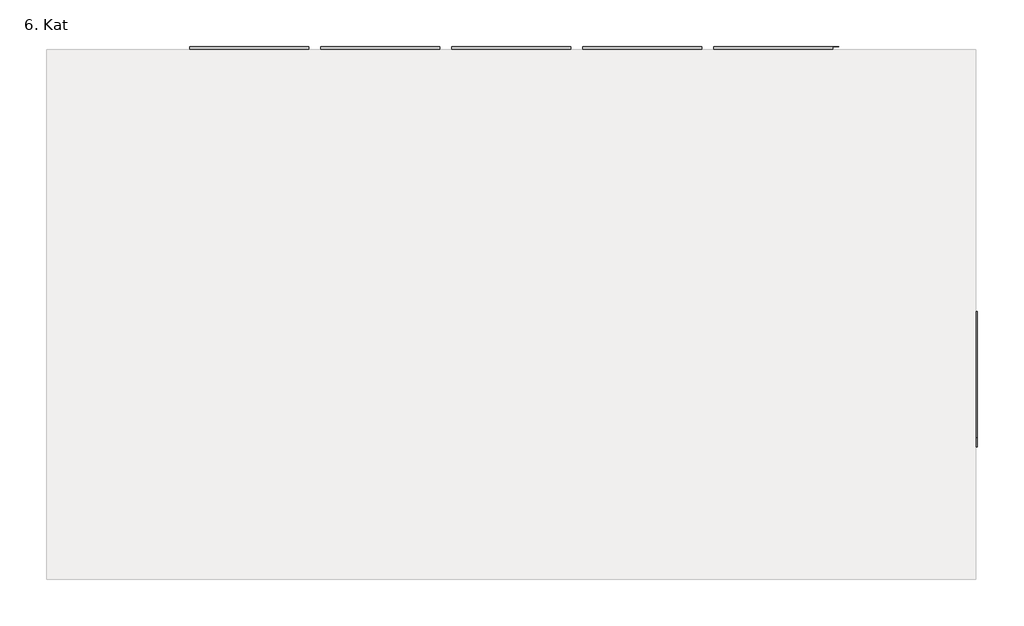
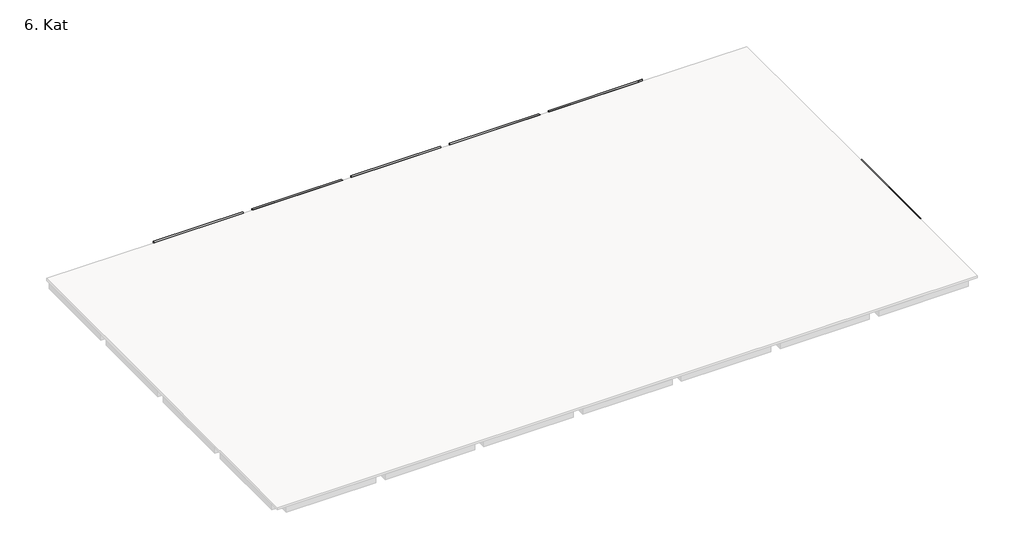
# One storey, part 2 of 2: 40 beams.
"""IFC4 building model written with IfcOpenShell, lengths in millimetres."""

from ifc_helpers import new_model, si_unit, frame, origin, place, context, project, spatial, polyline, outline, extrude, faceted_brep, element, save

model = new_model("IFC4")

# Units and contexts
model_context = context("Model", 3, world=origin())
ifc_project = project(units=[si_unit("LENGTHUNIT", "METRE", prefix="MILLI")], contexts=[model_context])

# Site, building, storey
site = spatial("IfcSite", under=ifc_project)
building = spatial("IfcBuilding", under=site)
storey = spatial("IfcBuildingStorey", under=building, Name="6. Kat", Elevation=31100.0)

# Beams
placement = place(None, origin())
element("IfcBeam", 1, ObjectType="M_Concrete-Rectangular Beam : 60x70cm kiriş", at=placement, inside=storey, context=model_context, shape_type="Brep", body=[
    faceted_brep([(16599.9993907, 34000.0004302, 31100.0), (16599.9993907, 34200.0000099, 31100.0), (8899.9995273, 34200.0000099, 31100.0), (8899.9995273, 34000.0004302, 31100.0), (8899.9993907, 33600.0000099, 30900.0), (8899.9993907, 33600.0000099, 30400.0), (16599.9993907, 33600.0000099, 30400.0), (16599.9993907, 33600.0000099, 30900.0), (8899.9995273, 34200.0000099, 30400.0), (16599.9993907, 34200.0000099, 30400.0), (8899.9993907, 34000.0004302, 30900.0), (16599.9993907, 34000.0004302, 30900.0)], [[[0, 1, 2, 3]], [[4, 5, 6, 7]], [[5, 8, 9, 6]], [[1, 9, 8, 2]], [[5, 4, 10, 3, 2, 8]], [[4, 7, 11, 10]], [[6, 9, 1, 0, 11, 7]], [[10, 11, 0, 3]]]),
])
element("IfcBeam", 2, ObjectType="M_Concrete-Rectangular Beam : 60x70cm kiriş", at=placement, inside=storey, context=model_context, shape_type="Brep", body=[
    faceted_brep([(25099.9993907, 34000.0004302, 31100.0), (25099.9993907, 34200.0000277, 31100.0), (17399.9993907, 34200.0000277, 31100.0), (17399.9993907, 34000.0004302, 31100.0), (25099.9993907, 33600.0000277, 30900.0), (17399.9996817, 33600.0000277, 30900.0), (17399.9996817, 33600.0000277, 30400.0), (25099.9993907, 33600.0000277, 30400.0), (17399.9993907, 34200.0000277, 30400.0), (25099.9993907, 34200.0000277, 30400.0), (17399.9993907, 34000.0004302, 30900.0), (25099.9993907, 34000.0004302, 30900.0)], [[[0, 1, 2, 3]], [[4, 5, 6, 7]], [[7, 6, 8, 9]], [[1, 9, 8, 2]], [[10, 5, 4, 11]], [[11, 0, 3, 10]], [[6, 5, 10, 3, 2, 8]], [[7, 9, 1, 0, 11, 4]]]),
])
element("IfcBeam", 3, ObjectType="M_Concrete-Rectangular Beam : 60x70cm kiriş", at=placement, inside=storey, context=model_context, shape_type="Brep", body=[
    faceted_brep([(33599.9993907, 34000.0004302, 31100.0), (33599.9993907, 34200.000044, 31100.0), (25899.9993907, 34200.000044, 31100.0), (25899.9993907, 34000.0004302, 31100.0), (33599.9993907, 34200.000044, 30400.0), (25899.9993907, 34200.000044, 30400.0), (25899.9996503, 33600.000044, 30400.0), (33599.9993907, 33600.000044, 30400.0), (25899.9996503, 33600.000044, 30900.0), (33599.9993907, 33600.000044, 30900.0), (25899.9993907, 34000.0004302, 30900.0), (33599.9993907, 34000.0004302, 30900.0)], [[[0, 1, 2, 3]], [[1, 4, 5, 2]], [[6, 5, 4, 7]], [[8, 6, 7, 9]], [[10, 8, 9, 11]], [[11, 0, 3, 10]], [[6, 8, 10, 3, 2, 5]], [[1, 0, 11, 9, 7, 4]]]),
])
element("IfcBeam", 4, ObjectType="M_Concrete-Rectangular Beam : 60x70cm kiriş", at=placement, inside=storey, context=model_context, shape_type="SweptSolid", body=[
    extrude(outline(polyline([(34200.0000618, 31100.0), (34200.0000618, 30400.0), (33600.0000618, 30400.0), (33600.0000618, 30900.0), (34000.0004302, 30900.0), (34000.0004302, 31100.0), (34200.0000618, 31100.0)])), frame((34399.9993907, 0.0, 0.0), z_axis=(1.0, 0.0, 0.0), x_axis=(0.0, 1.0, 0.0)), (0.0, 0.0, 1.0), 7699.9999993),
])
element("IfcBeam", 5, ObjectType="M_Concrete-Rectangular Beam : 60x70cm kiriş", at=placement, inside=storey, context=model_context, shape_type="Brep", body=[
    faceted_brep([(50999.9994944, 34200.0000788, 31100.0), (42899.999681, 34200.0000788, 31100.0), (42899.999681, 34000.0004302, 31100.0), (50599.9994944, 34000.0004302, 31100.0), (50599.9994944, 34193.7257565, 31100.0), (50999.9994944, 34193.7257565, 31100.0), (42899.999681, 34200.0000788, 30400.0), (50999.9994944, 34200.0000788, 30400.0), (42899.999681, 33600.0000788, 30400.0), (50999.9994944, 34193.7257565, 30400.0), (50599.9994944, 34193.7257565, 30400.0), (50599.9994944, 33600.0000788, 30400.0), (42899.999681, 33600.0000788, 30900.0), (50599.9994944, 33600.0000788, 30900.0), (42899.999681, 34000.0004302, 30900.0), (50599.9994944, 34000.0004302, 30900.0)], [[[0, 1, 2, 3, 4, 5]], [[6, 1, 0, 7]], [[8, 6, 7, 9, 10, 11]], [[12, 8, 11, 13]], [[14, 12, 13, 15]], [[2, 14, 15, 3]], [[1, 6, 8, 12, 14, 2]], [[7, 0, 5, 9]], [[10, 4, 3, 15, 13, 11]], [[4, 10, 9, 5]]]),
])
element("IfcBeam", 6, ObjectType="M_Concrete-Rectangular Beam : 60x70cm kiriş", at=placement, inside=storey, context=model_context, shape_type="SweptSolid", body=[
    extrude(outline(polyline([(16799.9996817, 33600.0009197), (17399.9996817, 33600.0009197), (17399.9996817, 25900.0003816), (16799.9996817, 25900.0003816), (16799.9996817, 33600.0009197)])), frame((0.0, 0.0, 30400.0), z_axis=(0.0, 0.0, 1.0), x_axis=(1.0, 0.0, 0.0)), (0.0, 0.0, 1.0), 500.0),
])
element("IfcBeam", 7, ObjectType="M_Concrete-Rectangular Beam : 60x70cm kiriş", at=placement, inside=storey, context=model_context, shape_type="SweptSolid", body=[
    extrude(outline(polyline([(25899.9996503, 25900.0004105), (25299.9996503, 25900.0004105), (25299.9996503, 33600.0009197), (25899.9996503, 33600.0009197), (25899.9996503, 25900.0004105)])), frame((0.0, 0.0, 30400.0), z_axis=(0.0, 0.0, 1.0), x_axis=(1.0, 0.0, 0.0)), (0.0, 0.0, 1.0), 500.0),
])
element("IfcBeam", 8, ObjectType="M_Concrete-Rectangular Beam : 60x70cm kiriş", at=placement, inside=storey, context=model_context, shape_type="Brep", body=[
    faceted_brep([(17399.9996817, 25900.0000279, 30400.0), (17399.9996817, 25900.0000279, 30900.0), (25099.9993907, 25900.0000279, 30900.0), (25099.9993907, 25900.0000279, 30400.0), (17399.9995362, 25300.0000279, 30400.0), (25099.9993907, 25300.0000279, 30400.0), (25099.9993907, 25300.0000279, 30900.0), (17399.9995362, 25300.0000279, 30900.0)], [[[0, 1, 2, 3]], [[4, 0, 3, 5]], [[5, 6, 7, 4]], [[4, 7, 1, 0]], [[2, 1, 7, 6]], [[5, 3, 2, 6]]]),
])
element("IfcBeam", 9, ObjectType="M_Concrete-Rectangular Beam : 60x70cm kiriş", at=placement, inside=storey, context=model_context, shape_type="SweptSolid", body=[
    extrude(outline(polyline([(25299.999682, 25099.9999518), (25899.999682, 25099.9999518), (25899.999682, 17400.0009197), (25299.999682, 17400.0009197), (25299.999682, 25099.9999518)])), frame((0.0, 0.0, 30400.0), z_axis=(0.0, 0.0, 1.0), x_axis=(1.0, 0.0, 0.0)), (0.0, 0.0, 1.0), 500.0),
])
element("IfcBeam", 10, ObjectType="M_Concrete-Rectangular Beam : 60x70cm kiriş", at=placement, inside=storey, context=model_context, shape_type="Brep", body=[
    faceted_brep([(25899.9996503, 25900.0003995, 30400.0), (25899.9996503, 25900.0003995, 30900.0), (33599.9993907, 25900.0003995, 30900.0), (33599.9993907, 25900.0003995, 30400.0), (25899.9993907, 25300.0003995, 30400.0), (33599.9993907, 25300.0003995, 30400.0), (25899.9993907, 25300.0003995, 30900.0), (33599.9993907, 25300.0003995, 30900.0)], [[[0, 1, 2, 3]], [[4, 0, 3, 5]], [[6, 4, 5, 7]], [[1, 0, 4, 6]], [[1, 6, 7, 2]], [[3, 2, 7, 5]]]),
])
element("IfcBeam", 11, ObjectType="M_Concrete-Rectangular Beam : 60x70cm kiriş", at=placement, inside=storey, context=model_context, shape_type="Brep", body=[
    faceted_brep([(33599.9994248, 33600.000044, 30900.0), (33599.9994248, 33600.000044, 30400.0), (33599.9994248, 25900.0003995, 30400.0), (33599.9994248, 25900.0003995, 30900.0), (34199.9994248, 33600.0009197, 30400.0), (34199.9994248, 25900.0004105, 30400.0), (34199.9994248, 25900.0004105, 30900.0), (34199.9994248, 33600.0009197, 30900.0)], [[[0, 1, 2, 3]], [[1, 4, 5, 2]], [[6, 5, 4, 7]], [[1, 0, 7, 4]], [[3, 2, 5, 6]], [[7, 0, 3, 6]]]),
])
element("IfcBeam", 12, ObjectType="M_Concrete-Rectangular Beam : 60x70cm kiriş", at=placement, inside=storey, context=model_context, shape_type="SweptSolid", body=[
    extrude(outline(polyline([(34399.9993907, 25300.0004179), (34399.9993907, 25900.0004179), (42099.9995162, 25900.0004179), (42099.9995162, 25300.0004179), (34399.9993907, 25300.0004179)])), frame((0.0, 0.0, 30400.0), z_axis=(0.0, 0.0, 1.0), x_axis=(1.0, 0.0, 0.0)), (0.0, 0.0, 1.0), 500.0),
])
element("IfcBeam", 13, ObjectType="M_Concrete-Rectangular Beam : 60x70cm kiriş", at=placement, inside=storey, context=model_context, shape_type="Brep", body=[
    faceted_brep([(42099.9994393, 25900.0004179, 30400.0), (42099.9994393, 25900.0004179, 30900.0), (42099.9994393, 33600.0000618, 30900.0), (42099.9994393, 33600.0000618, 30400.0), (42699.9994393, 25900.0004459, 30400.0), (42699.9994393, 33600.0009197, 30400.0), (42699.9994393, 33600.0009197, 30900.0), (42699.9994393, 25900.0004459, 30900.0)], [[[0, 1, 2, 3]], [[4, 0, 3, 5]], [[5, 6, 7, 4]], [[4, 7, 1, 0]], [[3, 2, 6, 5]], [[2, 1, 7, 6]]]),
])
element("IfcBeam", 14, ObjectType="M_Concrete-Rectangular Beam : 60x70cm kiriş", at=placement, inside=storey, context=model_context, shape_type="SweptSolid", body=[
    extrude(outline(polyline([(50599.9993899, 25900.0004722), (50599.9993899, 25300.0004722), (47199.999381, 25300.0004722), (47199.999381, 25900.0004722), (50599.9993899, 25900.0004722)])), frame((0.0, 0.0, 30400.0), z_axis=(0.0, 0.0, 1.0), x_axis=(1.0, 0.0, 0.0)), (0.0, 0.0, 1.0), 500.0),
])
element("IfcBeam", 15, ObjectType="M_Concrete-Rectangular Beam : 60x70cm kiriş", at=placement, inside=storey, context=model_context, shape_type="Brep", body=[
    faceted_brep([(51199.9994348, 25899.9999188, 30900.0), (51199.9994348, 25899.9999188, 30400.0), (51199.9994348, 33600.0004303, 30400.0), (51199.9994348, 33600.0004303, 30900.0), (50599.9994348, 33600.0000788, 30400.0), (50599.9994348, 25900.0004722, 30400.0), (50599.9994348, 33600.0000788, 30900.0), (50599.9994348, 25900.0004722, 30900.0)], [[[0, 1, 2, 3]], [[4, 2, 1, 5]], [[6, 4, 5, 7]], [[4, 6, 3, 2]], [[7, 5, 1, 0]], [[3, 6, 7, 0]]]),
])
element("IfcBeam", 16, ObjectType="M_Concrete-Rectangular Beam : 60x70cm kiriş", at=placement, inside=storey, context=model_context, shape_type="SweptSolid", body=[
    extrude(outline(polyline([(59100.0000836, 25300.0000972), (51399.9996879, 25300.0000972), (51399.9996879, 25900.0000972), (59100.0000836, 25900.0000972), (59100.0000836, 25300.0000972)])), frame((0.0, 0.0, 30400.0), z_axis=(0.0, 0.0, 1.0), x_axis=(1.0, 0.0, 0.0)), (0.0, 0.0, 1.0), 500.0),
])
element("IfcBeam", 17, ObjectType="M_Concrete-Rectangular Beam : 60x70cm kiriş", at=placement, inside=storey, context=model_context, shape_type="SweptSolid", body=[
    extrude(outline(polyline([(59899.9996867, 25900.0004522), (59299.9996867, 25900.0004522), (59299.9996867, 33600.0004303), (59899.9996867, 33600.0004303), (59899.9996867, 25900.0004522)])), frame((0.0, 0.0, 30400.0), z_axis=(0.0, 0.0, 1.0), x_axis=(1.0, 0.0, 0.0)), (0.0, 0.0, 1.0), 500.0),
])
element("IfcBeam", 18, ObjectType="M_Concrete-Rectangular Beam : 60x70cm kiriş", at=placement, inside=storey, context=model_context, shape_type="SweptSolid", body=[
    extrude(outline(polyline([(33599.9994953, 25100.0004105), (34199.9994953, 25100.0004105), (34199.9994953, 17400.0009197), (33599.9994953, 17400.0009197), (33599.9994953, 25100.0004105)])), frame((0.0, 0.0, 30400.0), z_axis=(0.0, 0.0, 1.0), x_axis=(1.0, 0.0, 0.0)), (0.0, 0.0, 1.0), 500.0),
])
element("IfcBeam", 19, ObjectType="M_Concrete-Rectangular Beam : 40x70cm kiriş 2", at=placement, inside=storey, context=model_context, shape_type="SweptSolid", body=[
    extrude(outline(polyline([(42099.9995162, 16050.0004138), (42499.9995162, 16050.0004138), (42499.9995162, 14100.0003816), (42099.9995162, 14100.0003816), (42099.9995162, 16050.0004138)])), frame((0.0, 0.0, 30400.0), z_axis=(0.0, 0.0, 1.0), x_axis=(1.0, 0.0, 0.0)), (0.0, 0.0, 1.0), 500.0),
])
element("IfcBeam", 20, ObjectType="M_Concrete-Rectangular Beam : 40x70cm kiriş 2", at=placement, inside=storey, context=model_context, shape_type="SweptSolid", body=[
    extrude(outline(polyline([(41999.9997966, 13700.0003995), (41999.9997966, 13300.0003995), (34399.9997415, 13300.0003995), (34399.9997415, 13700.0003995), (41999.9997966, 13700.0003995)])), frame((0.0, 0.0, 30400.0), z_axis=(0.0, 0.0, 1.0), x_axis=(1.0, 0.0, 0.0)), (0.0, 0.0, 1.0), 500.0),
])
element("IfcBeam", 21, ObjectType="M_Concrete-Rectangular Beam : 40x70cm kiriş 2", at=placement, inside=storey, context=model_context, shape_type="SweptSolid", body=[
    extrude(outline(polyline([(34399.9993907, 17000.0007895), (34399.9993907, 17400.0007895), (42099.9995162, 17400.0007895), (42099.9995162, 17000.0007895), (34399.9993907, 17000.0007895)])), frame((0.0, 0.0, 30400.0), z_axis=(0.0, 0.0, 1.0), x_axis=(1.0, 0.0, 0.0)), (0.0, 0.0, 1.0), 500.0),
])
element("IfcBeam", 22, ObjectType="M_Concrete-Rectangular Beam : 40x70cm kiriş 2", at=placement, inside=storey, context=model_context, shape_type="SweptSolid", body=[
    extrude(outline(polyline([(42499.9995162, 17000.0003766), (42499.9995162, 17400.0003766), (46799.999381, 17400.0003766), (46799.999381, 17000.0003766), (42499.9995162, 17000.0003766)])), frame((0.0, 0.0, 30400.0), z_axis=(0.0, 0.0, 1.0), x_axis=(1.0, 0.0, 0.0)), (0.0, 0.0, 1.0), 500.0),
])
element("IfcBeam", 23, ObjectType="M_Concrete-Rectangular Beam : 60x70cm kiriş", at=placement, inside=storey, context=model_context, shape_type="SweptSolid", body=[
    extrude(outline(polyline([(33599.9997451, 14100.0003995), (33599.9997451, 16599.9999518), (34199.9997451, 16599.9999518), (34199.9997451, 14100.0003995), (33599.9997451, 14100.0003995)])), frame((0.0, 0.0, 30400.0), z_axis=(0.0, 0.0, 1.0), x_axis=(1.0, 0.0, 0.0)), (0.0, 0.0, 1.0), 500.0),
])
element("IfcBeam", 24, ObjectType="M_Concrete-Rectangular Beam : 40x70cm kiriş 2", at=placement, inside=storey, context=model_context, shape_type="Brep", body=[
    faceted_brep([(42899.9990901, 13300.0003995, 30400.0), (46799.999381, 13300.0003995, 30400.0), (47199.999381, 13300.0003995, 30400.0), (50599.9996909, 13300.0003995, 30400.0), (50599.9996909, 13300.0003995, 30900.0), (47199.999381, 13300.0003995, 30900.0), (46799.999381, 13300.0003995, 30900.0), (42899.9990901, 13300.0003995, 30900.0), (42899.9990901, 13700.0003995, 30400.0), (46799.999381, 13700.0003995, 30400.0), (47199.999381, 13700.0003995, 30400.0), (50599.9996909, 13700.0003995, 30400.0), (42899.9990901, 13700.0003995, 30900.0), (46799.999381, 13700.0003995, 30900.0), (47199.999381, 13700.0003995, 30900.0), (50599.9996909, 13700.0003995, 30900.0)], [[[0, 1, 2, 3, 4, 5, 6, 7]], [[3, 2, 1, 0, 8, 9, 10, 11]], [[11, 10, 9, 8, 12, 13, 14, 15]], [[3, 11, 15, 4]], [[7, 6, 5, 4, 15, 14, 13, 12]], [[8, 0, 7, 12]]]),
])
element("IfcBeam", 25, ObjectType="M_Concrete-Rectangular Beam : 40x70cm kiriş 2", at=placement, inside=storey, context=model_context, shape_type="SweptSolid", body=[
    extrude(outline(polyline([(46799.999381, 16050.0004138), (47199.999381, 16050.0004138), (47199.999381, 13700.0003995), (46799.999381, 13700.0003995), (46799.999381, 16050.0004138)])), frame((0.0, 0.0, 30400.0), z_axis=(0.0, 0.0, 1.0), x_axis=(1.0, 0.0, 0.0)), (0.0, 0.0, 1.0), 500.0),
    extrude(outline(polyline([(46799.999381, 13300.0003995), (47199.999381, 13300.0003995), (47199.999381, 8800.0009197), (46799.999381, 8800.0009197), (46799.999381, 13300.0003995)])), frame((0.0, 0.0, 30400.0), z_axis=(0.0, 0.0, 1.0), x_axis=(1.0, 0.0, 0.0)), (0.0, 0.0, 1.0), 500.0),
])
element("IfcBeam", 26, ObjectType="M_Concrete-Rectangular Beam : 60x70cm kiriş", at=placement, inside=storey, context=model_context, shape_type="Brep", body=[
    faceted_brep([(34399.9993907, 8200.0009197, 30900.0), (34399.9993907, 8200.0009197, 30400.0), (42099.9993899, 8200.0009197, 30400.0), (42099.9993899, 8200.0009197, 30900.0), (34399.9993907, 8800.0009197, 30400.0), (41999.9997966, 8800.0009197, 30400.0), (42099.9993899, 8800.0009197, 30400.0), (34399.9993907, 8800.0009197, 30900.0), (41999.9997966, 8800.0009197, 30900.0), (42099.9993899, 8800.0009197, 30900.0)], [[[0, 1, 2, 3]], [[1, 4, 5, 6, 2]], [[4, 7, 8, 9, 6, 5]], [[7, 0, 3, 9, 8]], [[1, 0, 7, 4]], [[3, 2, 6, 9]]]),
])
element("IfcBeam", 27, ObjectType="M_Concrete-Rectangular Beam : 60x70cm kiriş", at=placement, inside=storey, context=model_context, shape_type="Brep", body=[
    faceted_brep([(50599.9993899, 8200.0009197, 30400.0), (50599.9993899, 8200.0009197, 30900.0), (42899.9993899, 8200.0009197, 30900.0), (42899.9993899, 8200.0009197, 30400.0), (50599.9993899, 8800.0009197, 30400.0), (42899.9993899, 8800.0009197, 30400.0), (46799.999381, 8800.0009197, 30400.0), (47199.999381, 8800.0009197, 30400.0), (50599.9993899, 8800.0009197, 30900.0), (42899.9993899, 8800.0009197, 30900.0), (46799.999381, 8800.0009197, 30900.0), (47199.999381, 8800.0009197, 30900.0)], [[[0, 1, 2, 3]], [[4, 0, 3, 5, 6, 7]], [[8, 4, 7, 6, 5, 9, 10, 11]], [[1, 8, 11, 10, 9, 2]], [[1, 0, 4, 8]], [[3, 2, 9, 5]]]),
])
element("IfcBeam", 28, ObjectType="M_Concrete-Rectangular Beam : 60x70cm kiriş", at=placement, inside=storey, context=model_context, shape_type="Brep", body=[
    faceted_brep([(42599.9997966, 8900.0009197, 30900.0), (42599.9997966, 8900.0009197, 30400.0), (42599.9997966, 13300.0003816, 30400.0), (42599.9997966, 13300.0003816, 30900.0), (41999.9997966, 8800.0009197, 30400.0), (41999.9997966, 13300.0003995, 30400.0), (41999.9997966, 13700.0003995, 30400.0), (42099.9993899, 13700.0003995, 30400.0), (42099.9993899, 13300.0003816, 30400.0), (42099.9993899, 8900.0009197, 30400.0), (42099.9993899, 8800.0009197, 30400.0), (41999.9997966, 8800.0009197, 30900.0), (41999.9997966, 13300.0003995, 30900.0), (41999.9997966, 13700.0003995, 30900.0), (42099.9993899, 8800.0009197, 30900.0), (42099.9993899, 8900.0009197, 30900.0), (42099.9993899, 13300.0003816, 30900.0), (42099.9993899, 13700.0003995, 30900.0)], [[[0, 1, 2, 3]], [[4, 5, 6, 7, 8, 2, 1, 9, 10]], [[4, 11, 12, 13, 6, 5]], [[11, 4, 10, 14]], [[13, 12, 11, 14, 15, 0, 3, 16, 17]], [[6, 13, 17, 7]], [[9, 15, 14, 10]], [[15, 9, 1, 0]], [[8, 16, 3, 2]], [[16, 8, 7, 17]]]),
])
element("IfcBeam", 29, ObjectType="M_Concrete-Rectangular Beam : 60x70cm kiriş", at=placement, inside=storey, context=model_context, shape_type="SweptSolid", body=[
    extrude(outline(polyline([(33599.9994953, 13300.0003995), (34199.9994953, 13300.0003995), (34199.9994953, 8900.0009197), (33599.9994953, 8900.0009197), (33599.9994953, 13300.0003995)])), frame((0.0, 0.0, 30400.0), z_axis=(0.0, 0.0, 1.0), x_axis=(1.0, 0.0, 0.0)), (0.0, 0.0, 1.0), 500.0),
])
element("IfcBeam", 30, ObjectType="M_Concrete-Rectangular Beam : 60x70cm kiriş", at=placement, inside=storey, context=model_context, shape_type="SweptSolid", body=[
    extrude(outline(polyline([(47199.999381, 16800.0008288), (47199.999381, 17400.0008288), (50599.9993899, 17400.0008288), (50599.9993899, 16800.0008288), (47199.999381, 16800.0008288)])), frame((0.0, 0.0, 30400.0), z_axis=(0.0, 0.0, 1.0), x_axis=(1.0, 0.0, 0.0)), (0.0, 0.0, 1.0), 500.0),
])
element("IfcBeam", 31, ObjectType="M_Concrete-Rectangular Beam : 60x70cm kiriş", at=placement, inside=storey, context=model_context, shape_type="Brep", body=[
    faceted_brep([(50599.999688, 17400.0008288, 30400.0), (50599.999688, 17400.0008288, 30900.0), (50599.999688, 25099.9999414, 30900.0), (50599.999688, 25099.9999414, 30400.0), (51199.999688, 17400.0009197, 30400.0), (51199.999688, 25099.9999414, 30400.0), (51199.999688, 25099.9999414, 30900.0), (51199.999688, 17400.0009197, 30900.0)], [[[0, 1, 2, 3]], [[4, 0, 3, 5]], [[5, 6, 7, 4]], [[4, 7, 1, 0]], [[2, 1, 7, 6]], [[5, 3, 2, 6]]]),
])
element("IfcBeam", 32, ObjectType="M_Concrete-Rectangular Beam : 60x70cm kiriş", at=placement, inside=storey, context=model_context, shape_type="SweptSolid", body=[
    extrude(outline(polyline([(59299.9997153, 17400.0009197), (59299.9997153, 25099.9999188), (59899.9997153, 25099.9999188), (59899.9997153, 17400.0009197), (59299.9997153, 17400.0009197)])), frame((0.0, 0.0, 30400.0), z_axis=(0.0, 0.0, 1.0), x_axis=(1.0, 0.0, 0.0)), (0.0, 0.0, 1.0), 500.0),
])
element("IfcBeam", 33, ObjectType="M_Concrete-Rectangular Beam : 60x70cm kiriş", at=placement, inside=storey, context=model_context, shape_type="SweptSolid", body=[
    extrude(outline(polyline([(51399.9993899, 17399.9995872), (59100.0000836, 17399.9995872), (59100.0000836, 16799.9995872), (51399.9993899, 16799.9995872), (51399.9993899, 17399.9995872)])), frame((0.0, 0.0, 30400.0), z_axis=(0.0, 0.0, 1.0), x_axis=(1.0, 0.0, 0.0)), (0.0, 0.0, 1.0), 500.0),
])
element("IfcBeam", 34, ObjectType="M_Concrete-Rectangular Beam : 60x70cm kiriş", at=placement, inside=storey, context=model_context, shape_type="Brep", body=[
    faceted_brep([(50599.9996909, 16600.0009197, 30400.0), (50599.9996909, 13700.0003995, 30400.0), (50599.9996909, 13300.0003995, 30400.0), (50599.9996909, 8900.000455, 30400.0), (50599.9996909, 8900.000455, 30900.0), (50599.9996909, 13300.0003995, 30900.0), (50599.9996909, 13700.0003995, 30900.0), (50599.9996909, 16600.0009197, 30900.0), (51199.9996909, 16600.0009197, 30400.0), (51199.9996909, 8900.000455, 30400.0), (51199.9996909, 16600.0009197, 30900.0), (51199.9996909, 8900.000455, 30900.0)], [[[0, 1, 2, 3, 4, 5, 6, 7]], [[3, 2, 1, 0, 8, 9]], [[9, 8, 10, 11]], [[7, 6, 5, 4, 11, 10]], [[3, 9, 11, 4]], [[8, 0, 7, 10]]]),
])
element("IfcBeam", 35, ObjectType="M_Concrete-Rectangular Beam : 60x70cm kiriş", at=placement, inside=storey, context=model_context, shape_type="Brep", body=[
    faceted_brep([(59999.9993848, 8200.0009197, 31100.0), (59999.9993848, 8800.0009197, 31100.0), (59899.9997758, 8800.0009197, 31100.0), (59899.9997758, 8200.0009197, 31100.0), (59999.9993848, 8200.0009197, 30400.0), (59900.0000836, 8200.0009197, 30400.0), (59999.9993848, 8800.0009197, 30400.0), (59900.0000836, 8800.0009197, 30400.0)], [[[0, 1, 2, 3]], [[4, 0, 3, 5]], [[6, 4, 5, 7]], [[1, 6, 7, 2]], [[1, 0, 4, 6]], [[3, 2, 7, 5]]]),
    faceted_brep([(51399.9993899, 8800.0009197, 30900.0), (51399.9993899, 8200.0009197, 30900.0), (59100.0000836, 8200.0009197, 30900.0), (59100.0000836, 8800.0009197, 30900.0), (51399.9993899, 8800.0009197, 30400.0), (51399.9993899, 8200.0009197, 30400.0), (59100.0000836, 8200.0009197, 30400.0), (59100.0000836, 8800.0009197, 30400.0)], [[[0, 1, 2, 3]], [[4, 5, 1, 0]], [[2, 6, 7, 3]], [[1, 5, 6, 2]], [[5, 4, 7, 6]], [[4, 0, 3, 7]]]),
])
element("IfcBeam", 36, ObjectType="M_Concrete-Rectangular Beam : 60x70cm kiriş", at=placement, inside=storey, context=model_context, shape_type="Brep", body=[
    faceted_brep([(59999.9993848, 8800.0009197, 31100.0), (59999.9993848, 17000.0009197, 31100.0), (59899.9997758, 17000.0009197, 31100.0), (59899.9997758, 8800.0009197, 31100.0), (59999.9993848, 17000.0009197, 30400.0), (59999.9993848, 8800.0009197, 30400.0), (59900.0000836, 8800.0009197, 30400.0), (59900.0000836, 8900.0009197, 30400.0), (59399.9993848, 8900.0009197, 30400.0), (59399.9993848, 16600.0009197, 30400.0), (59900.0000836, 16600.0009197, 30400.0), (59900.0000836, 17000.0009197, 30400.0), (59399.9993848, 8900.0009197, 30900.0), (59399.9993848, 16600.0009197, 30900.0), (59899.9997758, 8900.0009197, 30900.0), (59899.9997758, 16600.0009197, 30900.0)], [[[0, 1, 2, 3]], [[4, 1, 0, 5]], [[4, 5, 6, 7, 8, 9, 10, 11]], [[8, 12, 13, 9]], [[5, 0, 3, 6]], [[12, 14, 15, 13]], [[11, 10, 15, 14, 7, 6, 3, 2]], [[1, 4, 11, 2]], [[7, 14, 12, 8]], [[15, 10, 9, 13]]]),
])
element("IfcBeam", 37, ObjectType="M_Concrete-Rectangular Beam : 60x70cm kiriş", at=placement, inside=storey, context=model_context, shape_type="SweptSolid", body=[
    extrude(outline(polyline([(59899.9997503, 400.0009197), (59299.9997503, 400.0009197), (59299.9997503, 8100.0009197), (59899.9997503, 8100.0009197), (59899.9997503, 400.0009197)])), frame((0.0, 0.0, 30400.0), z_axis=(0.0, 0.0, 1.0), x_axis=(1.0, 0.0, 0.0)), (0.0, 0.0, 1.0), 500.0),
])
element("IfcBeam", 38, ObjectType="M_Concrete-Rectangular Beam : 60x70cm kiriş", at=placement, inside=storey, context=model_context, shape_type="SweptSolid", body=[
    extrude(outline(polyline([(51199.999723, 400.0009197), (50599.999723, 400.0009197), (50599.999723, 8100.0009197), (51199.999723, 8100.0009197), (51199.999723, 400.0009197)])), frame((0.0, 0.0, 30400.0), z_axis=(0.0, 0.0, 1.0), x_axis=(1.0, 0.0, 0.0)), (0.0, 0.0, 1.0), 500.0),
])
element("IfcBeam", 39, ObjectType="M_Concrete-Rectangular Beam : 60x70cm kiriş", at=placement, inside=storey, context=model_context, shape_type="SweptSolid", body=[
    extrude(outline(polyline([(42699.999723, 400.0009197), (42099.999723, 400.0009197), (42099.999723, 8100.0009197), (42699.999723, 8100.0009197), (42699.999723, 400.0009197)])), frame((0.0, 0.0, 30400.0), z_axis=(0.0, 0.0, 1.0), x_axis=(1.0, 0.0, 0.0)), (0.0, 0.0, 1.0), 500.0),
])
element("IfcBeam", 40, ObjectType="M_Concrete-Rectangular Beam : 60x70cm kiriş", at=placement, inside=storey, context=model_context, shape_type="SweptSolid", body=[
    extrude(outline(polyline([(33599.9997451, 400.0004179), (33599.9997451, 8100.0004174), (34199.9997451, 8100.0004174), (34199.9997451, 400.0004179), (33599.9997451, 400.0004179)])), frame((0.0, 0.0, 30400.0), z_axis=(0.0, 0.0, 1.0), x_axis=(1.0, 0.0, 0.0)), (0.0, 0.0, 1.0), 500.0),
])

save(model, "model.ifc")

# Revit data of these elements
# Type "M_Concrete-Rectangular Beam : 60x70cm kiriş"
#   Length [instance default] = 152.4 cm
#   b = 60 cm
#   h = 70 cm
#   Structural Material [instance default] = Concrete, Cast-in-Place gray
#   Assembly Code = ""
# Type "M_Concrete-Rectangular Beam : 40x70cm kiriş 2"
#   Length [instance default] = 152.4 cm
#   b = 40 cm
#   h = 70 cm
#   Structural Material [instance default] = Concrete, Cast-in-Place gray
#   Assembly Code = ""
# Elements 1, 2, 3, 4, 5, 6, 7, 8, 9, 10, 11, 12, 13, 14, 15, 16, 17, 18, 23, 26, 27, 28, 29, 30, 31, 32, 33, 34, 35, 36, 37, 38, 39, 40 (IfcBeam, "M_Concrete-Rectangular Beam : 60x70cm kiriş")
#   Comments = ""
#   Structural Material = Concrete, Cast-in-Place gray
#   Phase Created = New Construction
#   Materials on its faces: "Concrete, Cast-in-Place gray"
# Elements 19, 20, 21, 22, 24, 25 (IfcBeam, "M_Concrete-Rectangular Beam : 40x70cm kiriş 2")
#   Comments = ""
#   Structural Material = Concrete, Cast-in-Place gray
#   Phase Created = New Construction
#   Materials on its faces: "Concrete, Cast-in-Place gray"
# Materials
#   "Concrete, Cast-in-Place gray": class "Concrete", colour RGB 192 192 192, transparency 0, Description = "Cast-in-place concrete", Cost = 0
